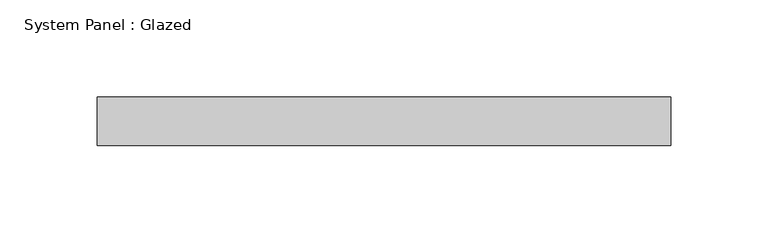
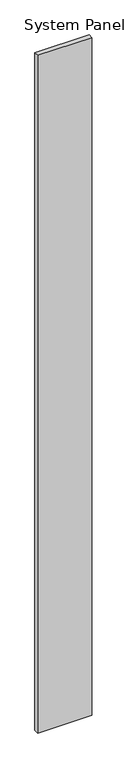
"""IFC4 building model written with IfcOpenShell, lengths in millimetres: plate geometry, System Panel : Glazed."""

import ifcopenshell
import ifcopenshell.guid

model = None  # the IFC model being written
_history = None  # IfcOwnerHistory: only IFC2X3 demands one
_inside = {}  # id of a spatial element -> (the spatial element, [elements in it])
_under = {}  # id of a project, library or spatial element -> (it, [spatial elements below it])
_declared = {}  # id of a project -> (the project, [libraries it declares])
_typed = {}  # id of a type object -> (the type object, [elements of that type])
_made_of = {}  # id of a material, layer set ... -> (it, [elements and type objects made of it])


def new_model(schema):
    """Start an empty IFC model of exactly this schema.

    Asked for "IFC4X3", IfcOpenShell would pick the latest addendum, in which some entities
    have other attributes; the version numbers below select the first issue.
    IFC2X3 requires an IfcOwnerHistory on every rooted entity: one is made here for all.
    """
    global model, _history
    if schema == "IFC4X3":
        model = ifcopenshell.file(schema_version=(4, 3, 0, 0))
    else:
        model = ifcopenshell.file(schema=schema)
    _inside.clear()
    _under.clear()
    _declared.clear()
    _typed.clear()
    _made_of.clear()
    _history = None
    if model.schema == "IFC2X3":
        org = make("IfcOrganization", Name="unknown")
        user = make(
            "IfcPersonAndOrganization",
            ThePerson=make("IfcPerson", FamilyName="unknown"),
            TheOrganization=org,
        )
        app = make(
            "IfcApplication",
            ApplicationDeveloper=org,
            Version="unknown",
            ApplicationFullName="unknown",
            ApplicationIdentifier="unknown",
        )
        _history = make(
            "IfcOwnerHistory",
            OwningUser=user,
            OwningApplication=app,
            ChangeAction="ADDED",
            CreationDate=0,
        )
    return model


def make(cls, **values):
    """One entity of the class cls with the attributes given. An attribute that is None is left unset."""
    return model.create_entity(
        cls, **{name: value for name, value in values.items() if value is not None}
    )


def rooted(cls, **values):
    """An entity with a GlobalId (a new one), such as an element, a storey or a relation."""
    return make(cls, GlobalId=ifcopenshell.guid.new(), OwnerHistory=_history, **values)


def si_unit(unit_type, name, prefix=None):
    """IfcSIUnit, for example si_unit("LENGTHUNIT", "METRE", prefix="MILLI")."""
    return make("IfcSIUnit", UnitType=unit_type, Prefix=prefix, Name=name)


def assignment(units):
    """IfcUnitAssignment: the units of a project."""
    return None if units is None else make("IfcUnitAssignment", Units=units)


def point(xyz):
    """IfcCartesianPoint."""
    return None if xyz is None else make("IfcCartesianPoint", Coordinates=xyz)


def direction(xyz):
    """IfcDirection."""
    return None if xyz is None else make("IfcDirection", DirectionRatios=xyz)


def frame(location, z_axis=None, x_axis=None):
    """IfcAxis2Placement3D, a coordinate frame: its origin and axes. An axis left out is left unset."""
    return make(
        "IfcAxis2Placement3D",
        Location=point(location),
        Axis=direction(z_axis),
        RefDirection=direction(x_axis),
    )


def origin():
    """The frame at (0, 0, 0) with its axes left unset."""
    return frame((0.0, 0.0, 0.0))


def origin_with_axes():
    """The frame at (0, 0, 0) with the z axis (0, 0, 1) and the x axis (1, 0, 0) written out."""
    return frame((0.0, 0.0, 0.0), z_axis=(0.0, 0.0, 1.0), x_axis=(1.0, 0.0, 0.0))


def place(relative_to, where):
    """IfcLocalPlacement: puts the frame where relative to a parent placement (None: the world)."""
    return make(
        "IfcLocalPlacement", PlacementRelTo=relative_to, RelativePlacement=where
    )


def context(
    kind, dimensions, precision=None, world=None, true_north=None, identifier=None
):
    """IfcGeometricRepresentationContext, for example the 3D "Model" context."""
    return make(
        "IfcGeometricRepresentationContext",
        ContextIdentifier=identifier,
        ContextType=kind,
        CoordinateSpaceDimension=dimensions,
        Precision=precision,
        WorldCoordinateSystem=world,
        TrueNorth=true_north,
    )


def project(units=None, contexts=None):
    """IfcProject with its units and contexts."""
    return rooted(
        "IfcProject",
        Name="project",
        RepresentationContexts=contexts,
        UnitsInContext=assignment(units),
    )


def spatial(cls, under=None, at=None, **own):
    """A site, building, storey or space (cls), placed at a placement, below another one or the project."""
    s = rooted(cls, ObjectPlacement=at, **own)
    if under is not None:
        _under.setdefault(under.id(), (under, []))[1].append(s)
    return s


def polyline(points):
    """IfcPolyline through the points."""
    return make("IfcPolyline", Points=[point(p) for p in points])


def outline(outer, holes=None, kind="AREA"):
    """IfcArbitraryClosedProfileDef: a profile drawn as a closed curve; with holes, ...WithVoids."""
    if holes is None:
        return make("IfcArbitraryClosedProfileDef", ProfileType=kind, OuterCurve=outer)
    return make(
        "IfcArbitraryProfileDefWithVoids",
        ProfileType=kind,
        OuterCurve=outer,
        InnerCurves=holes,
    )


def extrude(swept, where, along, depth):
    """IfcExtrudedAreaSolid: the profile swept, set in the frame where, extruded along a direction by depth."""
    return make(
        "IfcExtrudedAreaSolid",
        SweptArea=swept,
        Position=where,
        ExtrudedDirection=direction(along),
        Depth=depth,
    )


def shape(context_of_items, identifier, shape_type, items):
    """IfcShapeRepresentation: the items that make up one representation, for example the "Body"."""
    return make(
        "IfcShapeRepresentation",
        ContextOfItems=context_of_items,
        RepresentationIdentifier=identifier,
        RepresentationType=shape_type,
        Items=items,
    )


def source(mapping_origin, context_of_items, identifier, shape_type, items):
    """IfcRepresentationMap: a shape defined once, which mapped items show again and again."""
    return make(
        "IfcRepresentationMap",
        MappingOrigin=mapping_origin,
        MappedRepresentation=shape(context_of_items, identifier, shape_type, items),
    )


def transform(
    local_origin,
    x_axis=None,
    y_axis=None,
    z_axis=None,
    scale=None,
    scale2=None,
    scale3=None,
    uniform=True,
):
    """IfcCartesianTransformationOperator3D, or its non-uniform kind. x_axis, y_axis, z_axis: its Axis1, 2, 3."""
    if uniform:
        return make(
            "IfcCartesianTransformationOperator3D",
            Axis1=direction(x_axis),
            Axis2=direction(y_axis),
            LocalOrigin=point(local_origin),
            Scale=scale,
            Axis3=direction(z_axis),
        )
    return make(
        "IfcCartesianTransformationOperator3DnonUniform",
        Axis1=direction(x_axis),
        Axis2=direction(y_axis),
        LocalOrigin=point(local_origin),
        Scale=scale,
        Axis3=direction(z_axis),
        Scale2=scale2,
        Scale3=scale3,
    )


def mapped(mapping_source, mapping_target):
    """IfcMappedItem: shows the shape of a source again, moved by a transform."""
    return make(
        "IfcMappedItem", MappingSource=mapping_source, MappingTarget=mapping_target
    )


def made_of(thing, what):
    """Note that an element or type object is made of a material, layer set ...; save() writes the relation."""
    if what is not None:
        _made_of.setdefault(what.id(), (what, []))[1].append(thing)
    return thing


def element(
    cls,
    number,
    at=None,
    inside=None,
    cuts=None,
    type_object=None,
    material=None,
    context=None,
    identifier="Body",
    shape_type=None,
    held_by="IfcProductDefinitionShape",
    body=None,
    shapes=None,
    **own,
):
    """One element of the class cls, such as IfcWall. Its Tag is "e" and its number.

    at: its placement. inside: the storey or other place that contains it. cuts: it is an
    opening in that element (IfcRelVoidsElement). A single representation is given by context,
    identifier, shape_type and body (its items); several are given by shapes. held_by: the class
    of the entity that holds the representations. save() writes the other relations.
    """
    e = rooted(cls, Tag="e%d" % number, ObjectPlacement=at, **own)
    if body is not None:
        shapes = [shape(context, identifier, shape_type, body)]
    if shapes is not None:
        e.Representation = make(held_by, Representations=shapes)
    if inside is not None:
        _inside.setdefault(inside.id(), (inside, []))[1].append(e)
    if cuts is not None:
        rooted(
            "IfcRelVoidsElement", RelatingBuildingElement=cuts, RelatedOpeningElement=e
        )
    if type_object is not None:
        _typed.setdefault(type_object.id(), (type_object, []))[1].append(e)
    return made_of(e, material)


def aggregate(whole, parts):
    """IfcRelAggregates: a whole, such as a stair, and the parts it consists of."""
    return rooted("IfcRelAggregates", RelatingObject=whole, RelatedObjects=parts)


def save(model, path):
    """Write the relations noted so far, then the file.

    IfcRelAggregates (storeys below a building ...), IfcRelContainedInSpatialStructure (elements
    in a storey), IfcRelDefinesByType, IfcRelAssociatesMaterial and IfcRelDeclares: one each for
    every whole, place, type object, material and project.
    """
    for whole, parts in _under.values():
        aggregate(whole, parts)
    for where, things in _inside.values():
        rooted(
            "IfcRelContainedInSpatialStructure",
            RelatedElements=things,
            RelatingStructure=where,
        )
    for kind, things in _typed.values():
        rooted("IfcRelDefinesByType", RelatedObjects=things, RelatingType=kind)
    for what, things in _made_of.values():
        rooted("IfcRelAssociatesMaterial", RelatedObjects=things, RelatingMaterial=what)
    for by, libraries in _declared.values():
        rooted("IfcRelDeclares", RelatingContext=by, RelatedDefinitions=libraries)
    model.write(path)


def system_panel_glazed_71613ee9(model_context):
    return source(origin(), model_context, "Body", "SweptSolid", [
        extrude(outline(polyline([(147.4999998, 24.5), (-147.4999998, 24.5), (-147.4999998, 49.5), (147.4999998, 49.5), (147.4999998, 24.5)])), origin_with_axes(), (0.0, 0.0, 1.0), 3900.0),
    ])


if __name__ == "__main__":
    model = new_model("IFC4")
    model_context = context("Model", 3, world=origin())
    ifc_project = project(units=[si_unit("LENGTHUNIT", "METRE", prefix="MILLI")], contexts=[model_context])
    site = spatial("IfcSite", under=ifc_project)
    building = spatial("IfcBuilding", under=site)
    placement = place(None, origin())
    system_panel_glazed_shape = system_panel_glazed_71613ee9(model_context)
    element("IfcPlate", 1, ObjectType="System Panel : Glazed", at=placement, inside=building, context=model_context, shape_type="MappedRepresentation", body=[
        mapped(system_panel_glazed_shape, transform((0.0, 0.0, 0.0), x_axis=(1.0, 0.0, 0.0), y_axis=(0.0, 1.0, 0.0), z_axis=(0.0, 0.0, 1.0))),
    ])
    save(model, "model.ifc")

# Revit data of these elements
# Type "System Panel : Glazed"
#   Keynote = "H11"
#   Construction Type Id = "GSP4R"
#   Analytic Construction = "1/8 in Pilkington single glazing"
#   Visual Light Transmittance = 0.9
#   Solar Heat Gain Coefficient = 0.86
#   Heat Transfer Coefficient (U) = 6.7069 W/(m²·K)
#   Define Thermal Properties by = 1
# Element 1 (IfcPlate, "System Panel : Glazed")
#   Materials on its faces: "Glass"
# Materials
#   "Glass": class "Glass", colour RGB 0 128 192, transparency 0.9, Description = "Soda Lime Glass", Cost = 0
